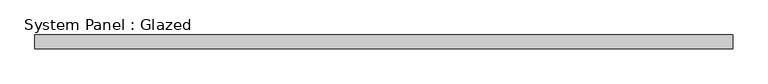
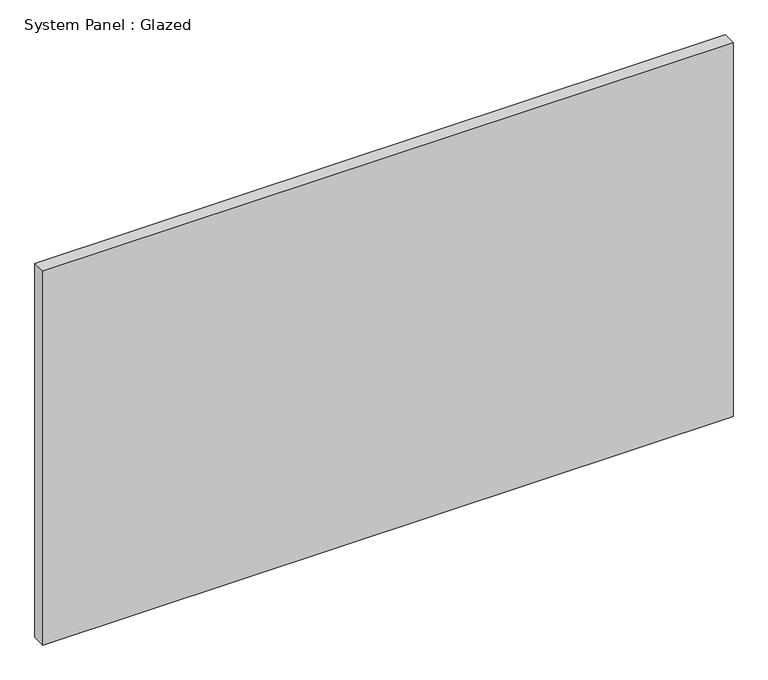
"""IFC4 building model written with IfcOpenShell, lengths in millimetres: plate geometry, System Panel : Glazed."""

import ifcopenshell
import ifcopenshell.guid

model = None  # the IFC model being written
_history = None  # IfcOwnerHistory: only IFC2X3 demands one
_inside = {}  # id of a spatial element -> (the spatial element, [elements in it])
_under = {}  # id of a project, library or spatial element -> (it, [spatial elements below it])
_declared = {}  # id of a project -> (the project, [libraries it declares])
_typed = {}  # id of a type object -> (the type object, [elements of that type])
_made_of = {}  # id of a material, layer set ... -> (it, [elements and type objects made of it])


def new_model(schema):
    """Start an empty IFC model of exactly this schema.

    Asked for "IFC4X3", IfcOpenShell would pick the latest addendum, in which some entities
    have other attributes; the version numbers below select the first issue.
    IFC2X3 requires an IfcOwnerHistory on every rooted entity: one is made here for all.
    """
    global model, _history
    if schema == "IFC4X3":
        model = ifcopenshell.file(schema_version=(4, 3, 0, 0))
    else:
        model = ifcopenshell.file(schema=schema)
    _inside.clear()
    _under.clear()
    _declared.clear()
    _typed.clear()
    _made_of.clear()
    _history = None
    if model.schema == "IFC2X3":
        org = make("IfcOrganization", Name="unknown")
        user = make(
            "IfcPersonAndOrganization",
            ThePerson=make("IfcPerson", FamilyName="unknown"),
            TheOrganization=org,
        )
        app = make(
            "IfcApplication",
            ApplicationDeveloper=org,
            Version="unknown",
            ApplicationFullName="unknown",
            ApplicationIdentifier="unknown",
        )
        _history = make(
            "IfcOwnerHistory",
            OwningUser=user,
            OwningApplication=app,
            ChangeAction="ADDED",
            CreationDate=0,
        )
    return model


def make(cls, **values):
    """One entity of the class cls with the attributes given. An attribute that is None is left unset."""
    return model.create_entity(
        cls, **{name: value for name, value in values.items() if value is not None}
    )


def rooted(cls, **values):
    """An entity with a GlobalId (a new one), such as an element, a storey or a relation."""
    return make(cls, GlobalId=ifcopenshell.guid.new(), OwnerHistory=_history, **values)


def si_unit(unit_type, name, prefix=None):
    """IfcSIUnit, for example si_unit("LENGTHUNIT", "METRE", prefix="MILLI")."""
    return make("IfcSIUnit", UnitType=unit_type, Prefix=prefix, Name=name)


def assignment(units):
    """IfcUnitAssignment: the units of a project."""
    return None if units is None else make("IfcUnitAssignment", Units=units)


def point(xyz):
    """IfcCartesianPoint."""
    return None if xyz is None else make("IfcCartesianPoint", Coordinates=xyz)


def direction(xyz):
    """IfcDirection."""
    return None if xyz is None else make("IfcDirection", DirectionRatios=xyz)


def frame(location, z_axis=None, x_axis=None):
    """IfcAxis2Placement3D, a coordinate frame: its origin and axes. An axis left out is left unset."""
    return make(
        "IfcAxis2Placement3D",
        Location=point(location),
        Axis=direction(z_axis),
        RefDirection=direction(x_axis),
    )


def origin():
    """The frame at (0, 0, 0) with its axes left unset."""
    return frame((0.0, 0.0, 0.0))


def origin_with_axes():
    """The frame at (0, 0, 0) with the z axis (0, 0, 1) and the x axis (1, 0, 0) written out."""
    return frame((0.0, 0.0, 0.0), z_axis=(0.0, 0.0, 1.0), x_axis=(1.0, 0.0, 0.0))


def place(relative_to, where):
    """IfcLocalPlacement: puts the frame where relative to a parent placement (None: the world)."""
    return make(
        "IfcLocalPlacement", PlacementRelTo=relative_to, RelativePlacement=where
    )


def context(
    kind, dimensions, precision=None, world=None, true_north=None, identifier=None
):
    """IfcGeometricRepresentationContext, for example the 3D "Model" context."""
    return make(
        "IfcGeometricRepresentationContext",
        ContextIdentifier=identifier,
        ContextType=kind,
        CoordinateSpaceDimension=dimensions,
        Precision=precision,
        WorldCoordinateSystem=world,
        TrueNorth=true_north,
    )


def project(units=None, contexts=None):
    """IfcProject with its units and contexts."""
    return rooted(
        "IfcProject",
        Name="project",
        RepresentationContexts=contexts,
        UnitsInContext=assignment(units),
    )


def spatial(cls, under=None, at=None, **own):
    """A site, building, storey or space (cls), placed at a placement, below another one or the project."""
    s = rooted(cls, ObjectPlacement=at, **own)
    if under is not None:
        _under.setdefault(under.id(), (under, []))[1].append(s)
    return s


def polyline(points):
    """IfcPolyline through the points."""
    return make("IfcPolyline", Points=[point(p) for p in points])


def outline(outer, holes=None, kind="AREA"):
    """IfcArbitraryClosedProfileDef: a profile drawn as a closed curve; with holes, ...WithVoids."""
    if holes is None:
        return make("IfcArbitraryClosedProfileDef", ProfileType=kind, OuterCurve=outer)
    return make(
        "IfcArbitraryProfileDefWithVoids",
        ProfileType=kind,
        OuterCurve=outer,
        InnerCurves=holes,
    )


def extrude(swept, where, along, depth):
    """IfcExtrudedAreaSolid: the profile swept, set in the frame where, extruded along a direction by depth."""
    return make(
        "IfcExtrudedAreaSolid",
        SweptArea=swept,
        Position=where,
        ExtrudedDirection=direction(along),
        Depth=depth,
    )


def shape(context_of_items, identifier, shape_type, items):
    """IfcShapeRepresentation: the items that make up one representation, for example the "Body"."""
    return make(
        "IfcShapeRepresentation",
        ContextOfItems=context_of_items,
        RepresentationIdentifier=identifier,
        RepresentationType=shape_type,
        Items=items,
    )


def source(mapping_origin, context_of_items, identifier, shape_type, items):
    """IfcRepresentationMap: a shape defined once, which mapped items show again and again."""
    return make(
        "IfcRepresentationMap",
        MappingOrigin=mapping_origin,
        MappedRepresentation=shape(context_of_items, identifier, shape_type, items),
    )


def transform(
    local_origin,
    x_axis=None,
    y_axis=None,
    z_axis=None,
    scale=None,
    scale2=None,
    scale3=None,
    uniform=True,
):
    """IfcCartesianTransformationOperator3D, or its non-uniform kind. x_axis, y_axis, z_axis: its Axis1, 2, 3."""
    if uniform:
        return make(
            "IfcCartesianTransformationOperator3D",
            Axis1=direction(x_axis),
            Axis2=direction(y_axis),
            LocalOrigin=point(local_origin),
            Scale=scale,
            Axis3=direction(z_axis),
        )
    return make(
        "IfcCartesianTransformationOperator3DnonUniform",
        Axis1=direction(x_axis),
        Axis2=direction(y_axis),
        LocalOrigin=point(local_origin),
        Scale=scale,
        Axis3=direction(z_axis),
        Scale2=scale2,
        Scale3=scale3,
    )


def mapped(mapping_source, mapping_target):
    """IfcMappedItem: shows the shape of a source again, moved by a transform."""
    return make(
        "IfcMappedItem", MappingSource=mapping_source, MappingTarget=mapping_target
    )


def made_of(thing, what):
    """Note that an element or type object is made of a material, layer set ...; save() writes the relation."""
    if what is not None:
        _made_of.setdefault(what.id(), (what, []))[1].append(thing)
    return thing


def element(
    cls,
    number,
    at=None,
    inside=None,
    cuts=None,
    type_object=None,
    material=None,
    context=None,
    identifier="Body",
    shape_type=None,
    held_by="IfcProductDefinitionShape",
    body=None,
    shapes=None,
    **own,
):
    """One element of the class cls, such as IfcWall. Its Tag is "e" and its number.

    at: its placement. inside: the storey or other place that contains it. cuts: it is an
    opening in that element (IfcRelVoidsElement). A single representation is given by context,
    identifier, shape_type and body (its items); several are given by shapes. held_by: the class
    of the entity that holds the representations. save() writes the other relations.
    """
    e = rooted(cls, Tag="e%d" % number, ObjectPlacement=at, **own)
    if body is not None:
        shapes = [shape(context, identifier, shape_type, body)]
    if shapes is not None:
        e.Representation = make(held_by, Representations=shapes)
    if inside is not None:
        _inside.setdefault(inside.id(), (inside, []))[1].append(e)
    if cuts is not None:
        rooted(
            "IfcRelVoidsElement", RelatingBuildingElement=cuts, RelatedOpeningElement=e
        )
    if type_object is not None:
        _typed.setdefault(type_object.id(), (type_object, []))[1].append(e)
    return made_of(e, material)


def aggregate(whole, parts):
    """IfcRelAggregates: a whole, such as a stair, and the parts it consists of."""
    return rooted("IfcRelAggregates", RelatingObject=whole, RelatedObjects=parts)


def save(model, path):
    """Write the relations noted so far, then the file.

    IfcRelAggregates (storeys below a building ...), IfcRelContainedInSpatialStructure (elements
    in a storey), IfcRelDefinesByType, IfcRelAssociatesMaterial and IfcRelDeclares: one each for
    every whole, place, type object, material and project.
    """
    for whole, parts in _under.values():
        aggregate(whole, parts)
    for where, things in _inside.values():
        rooted(
            "IfcRelContainedInSpatialStructure",
            RelatedElements=things,
            RelatingStructure=where,
        )
    for kind, things in _typed.values():
        rooted("IfcRelDefinesByType", RelatedObjects=things, RelatingType=kind)
    for what, things in _made_of.values():
        rooted("IfcRelAssociatesMaterial", RelatedObjects=things, RelatingMaterial=what)
    for by, libraries in _declared.values():
        rooted("IfcRelDeclares", RelatingContext=by, RelatedDefinitions=libraries)
    model.write(path)


def system_panel_glazed_8e5047c4(model_context):
    return source(origin(), model_context, "Body", "SweptSolid", [
        extrude(outline(polyline([(632.4999999, 24.5), (-632.4999999, 24.5), (-632.4999999, 49.5), (632.4999999, 49.5), (632.4999999, 24.5)])), origin_with_axes(), (0.0, 0.0, 1.0), 725.0),
    ])


if __name__ == "__main__":
    model = new_model("IFC4")
    model_context = context("Model", 3, world=origin())
    ifc_project = project(units=[si_unit("LENGTHUNIT", "METRE", prefix="MILLI")], contexts=[model_context])
    site = spatial("IfcSite", under=ifc_project)
    building = spatial("IfcBuilding", under=site)
    placement = place(None, origin())
    system_panel_glazed_shape = system_panel_glazed_8e5047c4(model_context)
    element("IfcPlate", 1, ObjectType="System Panel : Glazed", at=placement, inside=building, context=model_context, shape_type="MappedRepresentation", body=[
        mapped(system_panel_glazed_shape, transform((0.0, 0.0, 0.0), x_axis=(1.0, 0.0, 0.0), y_axis=(0.0, 1.0, 0.0), z_axis=(0.0, 0.0, 1.0))),
    ])
    save(model, "model.ifc")

# Revit data of these elements
# Type "System Panel : Glazed"
#   Construction Type Id = "GSP4R"
#   Analytic Construction = "1/8 in Pilkington single glazing"
#   Visual Light Transmittance = 0.9
#   Solar Heat Gain Coefficient = 0.86
#   Heat Transfer Coefficient (U) = 6.7069 W/(m²·K)
#   Define Thermal Properties by = 1
# Element 1 (IfcPlate, "System Panel : Glazed")
#   Materials on its faces: "Glass"
# Materials
#   "Glass": class "Glass", colour RGB 0 128 192, transparency 0.9, Description = "Soda Lime Glass", Cost = 0
